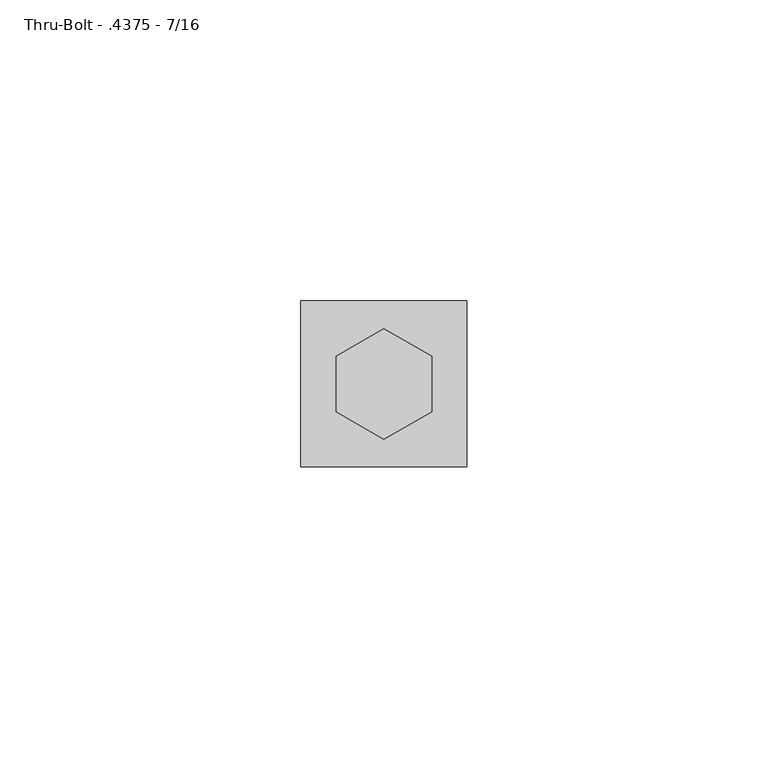
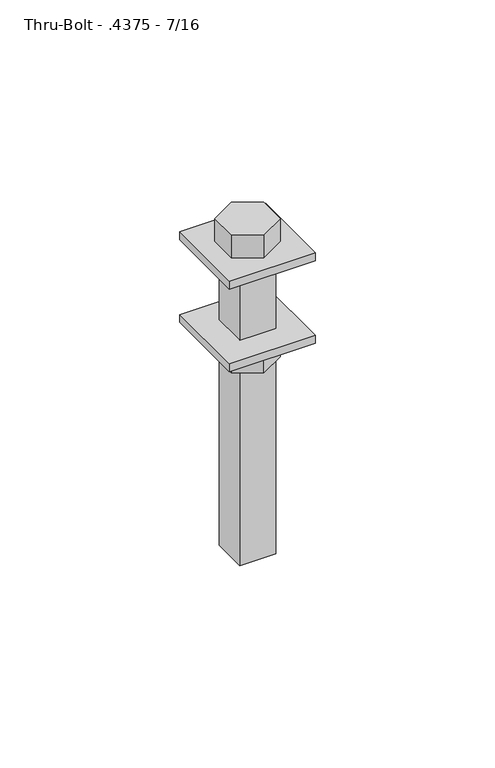
"""IFC4 building model written with IfcOpenShell, lengths in millimetres: fastener geometry, 060523 - W_P_C - Fastenings - Generic - SQUARE : Thru-Bolt - .4375 - 7/16."""

import ifcopenshell
import ifcopenshell.guid

model = None  # the IFC model being written
_history = None  # IfcOwnerHistory: only IFC2X3 demands one
_inside = {}  # id of a spatial element -> (the spatial element, [elements in it])
_under = {}  # id of a project, library or spatial element -> (it, [spatial elements below it])
_declared = {}  # id of a project -> (the project, [libraries it declares])
_typed = {}  # id of a type object -> (the type object, [elements of that type])
_made_of = {}  # id of a material, layer set ... -> (it, [elements and type objects made of it])


def new_model(schema):
    """Start an empty IFC model of exactly this schema.

    Asked for "IFC4X3", IfcOpenShell would pick the latest addendum, in which some entities
    have other attributes; the version numbers below select the first issue.
    IFC2X3 requires an IfcOwnerHistory on every rooted entity: one is made here for all.
    """
    global model, _history
    if schema == "IFC4X3":
        model = ifcopenshell.file(schema_version=(4, 3, 0, 0))
    else:
        model = ifcopenshell.file(schema=schema)
    _inside.clear()
    _under.clear()
    _declared.clear()
    _typed.clear()
    _made_of.clear()
    _history = None
    if model.schema == "IFC2X3":
        org = make("IfcOrganization", Name="unknown")
        user = make(
            "IfcPersonAndOrganization",
            ThePerson=make("IfcPerson", FamilyName="unknown"),
            TheOrganization=org,
        )
        app = make(
            "IfcApplication",
            ApplicationDeveloper=org,
            Version="unknown",
            ApplicationFullName="unknown",
            ApplicationIdentifier="unknown",
        )
        _history = make(
            "IfcOwnerHistory",
            OwningUser=user,
            OwningApplication=app,
            ChangeAction="ADDED",
            CreationDate=0,
        )
    return model


def make(cls, **values):
    """One entity of the class cls with the attributes given. An attribute that is None is left unset."""
    return model.create_entity(
        cls, **{name: value for name, value in values.items() if value is not None}
    )


def rooted(cls, **values):
    """An entity with a GlobalId (a new one), such as an element, a storey or a relation."""
    return make(cls, GlobalId=ifcopenshell.guid.new(), OwnerHistory=_history, **values)


def si_unit(unit_type, name, prefix=None):
    """IfcSIUnit, for example si_unit("LENGTHUNIT", "METRE", prefix="MILLI")."""
    return make("IfcSIUnit", UnitType=unit_type, Prefix=prefix, Name=name)


def assignment(units):
    """IfcUnitAssignment: the units of a project."""
    return None if units is None else make("IfcUnitAssignment", Units=units)


def point(xyz):
    """IfcCartesianPoint."""
    return None if xyz is None else make("IfcCartesianPoint", Coordinates=xyz)


def direction(xyz):
    """IfcDirection."""
    return None if xyz is None else make("IfcDirection", DirectionRatios=xyz)


def frame(location, z_axis=None, x_axis=None):
    """IfcAxis2Placement3D, a coordinate frame: its origin and axes. An axis left out is left unset."""
    return make(
        "IfcAxis2Placement3D",
        Location=point(location),
        Axis=direction(z_axis),
        RefDirection=direction(x_axis),
    )


def origin():
    """The frame at (0, 0, 0) with its axes left unset."""
    return frame((0.0, 0.0, 0.0))


def origin_with_axes():
    """The frame at (0, 0, 0) with the z axis (0, 0, 1) and the x axis (1, 0, 0) written out."""
    return frame((0.0, 0.0, 0.0), z_axis=(0.0, 0.0, 1.0), x_axis=(1.0, 0.0, 0.0))


def place(relative_to, where):
    """IfcLocalPlacement: puts the frame where relative to a parent placement (None: the world)."""
    return make(
        "IfcLocalPlacement", PlacementRelTo=relative_to, RelativePlacement=where
    )


def context(
    kind, dimensions, precision=None, world=None, true_north=None, identifier=None
):
    """IfcGeometricRepresentationContext, for example the 3D "Model" context."""
    return make(
        "IfcGeometricRepresentationContext",
        ContextIdentifier=identifier,
        ContextType=kind,
        CoordinateSpaceDimension=dimensions,
        Precision=precision,
        WorldCoordinateSystem=world,
        TrueNorth=true_north,
    )


def project(units=None, contexts=None):
    """IfcProject with its units and contexts."""
    return rooted(
        "IfcProject",
        Name="project",
        RepresentationContexts=contexts,
        UnitsInContext=assignment(units),
    )


def spatial(cls, under=None, at=None, **own):
    """A site, building, storey or space (cls), placed at a placement, below another one or the project."""
    s = rooted(cls, ObjectPlacement=at, **own)
    if under is not None:
        _under.setdefault(under.id(), (under, []))[1].append(s)
    return s


def polyline(points):
    """IfcPolyline through the points."""
    return make("IfcPolyline", Points=[point(p) for p in points])


def outline(outer, holes=None, kind="AREA"):
    """IfcArbitraryClosedProfileDef: a profile drawn as a closed curve; with holes, ...WithVoids."""
    if holes is None:
        return make("IfcArbitraryClosedProfileDef", ProfileType=kind, OuterCurve=outer)
    return make(
        "IfcArbitraryProfileDefWithVoids",
        ProfileType=kind,
        OuterCurve=outer,
        InnerCurves=holes,
    )


def extrude(swept, where, along, depth):
    """IfcExtrudedAreaSolid: the profile swept, set in the frame where, extruded along a direction by depth."""
    return make(
        "IfcExtrudedAreaSolid",
        SweptArea=swept,
        Position=where,
        ExtrudedDirection=direction(along),
        Depth=depth,
    )


def shape(context_of_items, identifier, shape_type, items):
    """IfcShapeRepresentation: the items that make up one representation, for example the "Body"."""
    return make(
        "IfcShapeRepresentation",
        ContextOfItems=context_of_items,
        RepresentationIdentifier=identifier,
        RepresentationType=shape_type,
        Items=items,
    )


def source(mapping_origin, context_of_items, identifier, shape_type, items):
    """IfcRepresentationMap: a shape defined once, which mapped items show again and again."""
    return make(
        "IfcRepresentationMap",
        MappingOrigin=mapping_origin,
        MappedRepresentation=shape(context_of_items, identifier, shape_type, items),
    )


def transform(
    local_origin,
    x_axis=None,
    y_axis=None,
    z_axis=None,
    scale=None,
    scale2=None,
    scale3=None,
    uniform=True,
):
    """IfcCartesianTransformationOperator3D, or its non-uniform kind. x_axis, y_axis, z_axis: its Axis1, 2, 3."""
    if uniform:
        return make(
            "IfcCartesianTransformationOperator3D",
            Axis1=direction(x_axis),
            Axis2=direction(y_axis),
            LocalOrigin=point(local_origin),
            Scale=scale,
            Axis3=direction(z_axis),
        )
    return make(
        "IfcCartesianTransformationOperator3DnonUniform",
        Axis1=direction(x_axis),
        Axis2=direction(y_axis),
        LocalOrigin=point(local_origin),
        Scale=scale,
        Axis3=direction(z_axis),
        Scale2=scale2,
        Scale3=scale3,
    )


def mapped(mapping_source, mapping_target):
    """IfcMappedItem: shows the shape of a source again, moved by a transform."""
    return make(
        "IfcMappedItem", MappingSource=mapping_source, MappingTarget=mapping_target
    )


def made_of(thing, what):
    """Note that an element or type object is made of a material, layer set ...; save() writes the relation."""
    if what is not None:
        _made_of.setdefault(what.id(), (what, []))[1].append(thing)
    return thing


def element(
    cls,
    number,
    at=None,
    inside=None,
    cuts=None,
    type_object=None,
    material=None,
    context=None,
    identifier="Body",
    shape_type=None,
    held_by="IfcProductDefinitionShape",
    body=None,
    shapes=None,
    **own,
):
    """One element of the class cls, such as IfcWall. Its Tag is "e" and its number.

    at: its placement. inside: the storey or other place that contains it. cuts: it is an
    opening in that element (IfcRelVoidsElement). A single representation is given by context,
    identifier, shape_type and body (its items); several are given by shapes. held_by: the class
    of the entity that holds the representations. save() writes the other relations.
    """
    e = rooted(cls, Tag="e%d" % number, ObjectPlacement=at, **own)
    if body is not None:
        shapes = [shape(context, identifier, shape_type, body)]
    if shapes is not None:
        e.Representation = make(held_by, Representations=shapes)
    if inside is not None:
        _inside.setdefault(inside.id(), (inside, []))[1].append(e)
    if cuts is not None:
        rooted(
            "IfcRelVoidsElement", RelatingBuildingElement=cuts, RelatedOpeningElement=e
        )
    if type_object is not None:
        _typed.setdefault(type_object.id(), (type_object, []))[1].append(e)
    return made_of(e, material)


def aggregate(whole, parts):
    """IfcRelAggregates: a whole, such as a stair, and the parts it consists of."""
    return rooted("IfcRelAggregates", RelatingObject=whole, RelatedObjects=parts)


def save(model, path):
    """Write the relations noted so far, then the file.

    IfcRelAggregates (storeys below a building ...), IfcRelContainedInSpatialStructure (elements
    in a storey), IfcRelDefinesByType, IfcRelAssociatesMaterial and IfcRelDeclares: one each for
    every whole, place, type object, material and project.
    """
    for whole, parts in _under.values():
        aggregate(whole, parts)
    for where, things in _inside.values():
        rooted(
            "IfcRelContainedInSpatialStructure",
            RelatedElements=things,
            RelatingStructure=where,
        )
    for kind, things in _typed.values():
        rooted("IfcRelDefinesByType", RelatedObjects=things, RelatingType=kind)
    for what, things in _made_of.values():
        rooted("IfcRelAssociatesMaterial", RelatedObjects=things, RelatingMaterial=what)
    for by, libraries in _declared.values():
        rooted("IfcRelDeclares", RelatingContext=by, RelatedDefinitions=libraries)
    model.write(path)


def thru_bolt_4375_7_16_bbfdf3dc(model_context):
    return source(origin(), model_context, "Body", "SweptSolid", [
        extrude(outline(polyline([(-13.7914063, -13.7914063), (-13.7914063, 13.7914062), (13.7914062, 13.7914062), (13.7914062, -13.7914063), (-13.7914063, -13.7914063)])), origin_with_axes(), (0.0, 0.0, 1.0), 2.6789062),
        extrude(outline(polyline([(-13.7914063, -13.7914063), (-13.7914063, 13.7914062), (13.7914062, 13.7914062), (13.7914062, -13.7914063), (-13.7914063, -13.7914063)])), frame((0.0, 0.0, -28.0789063), z_axis=(0.0, 0.0, 1.0), x_axis=(1.0, 0.0, 0.0)), (0.0, 0.0, 1.0), 2.6789062),
        extrude(outline(polyline([(-7.9375, -4.5827178), (-7.9375, 4.5827178), (0.0, 9.1654355), (7.9375, 4.5827178), (7.9375, -4.5827178), (0.0, -9.1654355), (-7.9375, -4.5827178)])), frame((0.0, 0.0, -36.115625), z_axis=(0.0, 0.0, 1.0), x_axis=(1.0, 0.0, 0.0)), (0.0, 0.0, 1.0), 8.0367187),
        extrude(outline(polyline([(-7.9375, 4.5827178), (0.0, 9.1654355), (7.9375, 4.5827178), (7.9375, -4.5827178), (0.0, -9.1654355), (-7.9375, -4.5827178), (-7.9375, 4.5827178)])), frame((0.0, 0.0, 2.6789063), z_axis=(0.0, 0.0, 1.0), x_axis=(1.0, 0.0, 0.0)), (0.0, 0.0, 1.0), 8.0367187),
        extrude(outline(polyline([(-5.7546875, 5.7546875), (5.7546875, 5.7546875), (5.7546875, -5.7546875), (-5.7546875, -5.7546875), (-5.7546875, 5.7546875)])), frame((0.0, 0.0, -101.6), z_axis=(0.0, 0.0, 1.0), x_axis=(1.0, 0.0, 0.0)), (0.0, 0.0, 1.0), 104.2789062),
    ])


if __name__ == "__main__":
    model = new_model("IFC4")
    model_context = context("Model", 3, world=origin())
    ifc_project = project(units=[si_unit("LENGTHUNIT", "METRE", prefix="MILLI")], contexts=[model_context])
    site = spatial("IfcSite", under=ifc_project)
    building = spatial("IfcBuilding", under=site)
    placement = place(None, origin())
    thru_bolt_4375_7_16_shape = thru_bolt_4375_7_16_bbfdf3dc(model_context)
    element("IfcFastener", 1, ObjectType="060523 - W_P_C - Fastenings - Generic - SQUARE : Thru-Bolt - .4375 - 7/16", at=placement, inside=building, context=model_context, shape_type="MappedRepresentation", body=[
        mapped(thru_bolt_4375_7_16_shape, transform((0.0, 0.0, 0.0), x_axis=(1.0, 0.0, 0.0), y_axis=(0.0, 1.0, 0.0), z_axis=(0.0, 0.0, 1.0))),
    ])
    save(model, "model.ifc")

# Revit data of these elements
# Type "060523 - W_P_C - Fastenings - Generic - SQUARE : Thru-Bolt - .4375 - 7/16"
#   Washer_Thickness = 0' - 0 27/256"
#   Washer Radius = 0' - 0 139/256"
#   Washer Offset - Head = 0' - 0 27/256"
#   Washer Offset = 0' - 0 27/256"
#   Thickness_of_Substrate [instance default] = 0' - 1"
#   Side = 0' - 0.36133"
#   Radius = 0' - 0 29/128"
#   Length [instance default] = 0' - 4"
#   Head Size = 0' - 0 5/8"
#   Head Radius = 0' - 0 5/16"
#   Head Height = 0' - 0 81/256"
#   Double Diameter = 0' - 0 29/32"
#   Diameter = 0' - 0 29/64"
#   Default Elevation = 4' - 0"
#   Washer_Nut_Visibility = yes
#   Washer_Head_Visibility = yes
#   Round_Head_Visibility = no
#   Point Visibility = no
#   Nut_Visibility = yes
#   Hex_Head_Visiblilty = yes
#   Washer Material = none
#   Bolt Material (Size) = AT SILL - FASTENER AT 24" O.C.
# Element 1 (IfcFastener, "060523 - W_P_C - Fastenings - Generic - SQUARE : Thru-Bolt - .4375 - 7/16")
#   Materials on its faces: "AT SILL - FASTENER AT 24\" O.C."
# Materials
#   "AT SILL - FASTENER AT 24\" O.C.": class "Generic", colour RGB 120 120 120, transparency 0, Cost = 0
